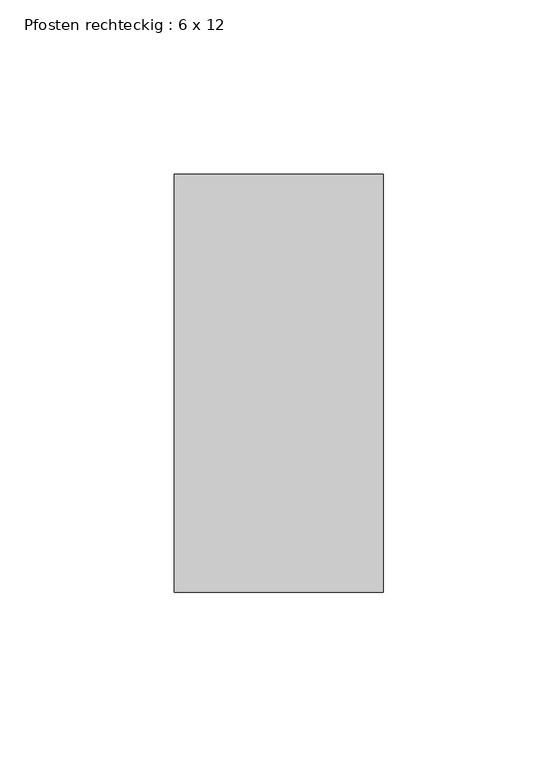
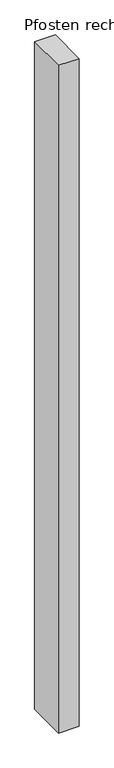
"""IFC4 building model written with IfcOpenShell, lengths in millimetres: member geometry, Pfosten rechteckig : 6 x 12."""

from ifc_helpers import new_model, si_unit, frame, origin, place, context, project, spatial, polyline, outline, extrude, source, transform, mapped, element, save


def pfosten_rechteckig_6_x_12_07c25811(model_context):
    return source(origin(), model_context, "Body", "SweptSolid", [
        extrude(outline(polyline([(30.0, 60.0), (30.0, -60.0), (-30.0, -60.0), (-30.0, 60.0), (30.0, 60.0)])), frame((0.0, 0.0, -2050.0000003), z_axis=(0.0, 0.0, 1.0), x_axis=(1.0, 0.0, 0.0)), (0.0, 0.0, 1.0), 2050.0000003),
    ])


if __name__ == "__main__":
    model = new_model("IFC4")
    model_context = context("Model", 3, world=origin())
    ifc_project = project(units=[si_unit("LENGTHUNIT", "METRE", prefix="MILLI")], contexts=[model_context])
    site = spatial("IfcSite", under=ifc_project)
    building = spatial("IfcBuilding", under=site)
    placement = place(None, origin())
    pfosten_rechteckig_6_x_12_shape = pfosten_rechteckig_6_x_12_07c25811(model_context)
    element("IfcMember", 1, ObjectType="Pfosten rechteckig : 6 x 12", at=placement, inside=building, context=model_context, shape_type="MappedRepresentation", body=[
        mapped(pfosten_rechteckig_6_x_12_shape, transform((0.0, 0.0, 0.0), x_axis=(1.0, 0.0, 0.0), y_axis=(0.0, 1.0, 0.0), z_axis=(0.0, 0.0, 1.0))),
    ])
    save(model, "model.ifc")

# Revit data of these elements
# Type "Pfosten rechteckig : 6 x 12"
#   built-in parameter 1007304 = 0.393701 (stored number, unit not read)
#   built-in parameter 1007301 = 0.0984252 (stored number, unit not read)
#   built-in parameter 1007300 = 0.0984252 (stored number, unit not read)
# Element 1 (IfcMember, "Pfosten rechteckig : 6 x 12")
#   Materials on its faces: "Metall - verzinkt"
# Materials
#   "Metall - verzinkt": class "Allgemeines", colour RGB 200 200 200, transparency 0, Cost = 0
